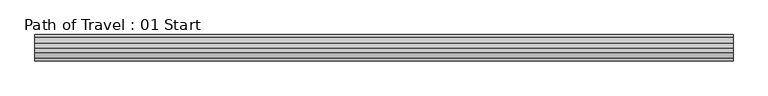
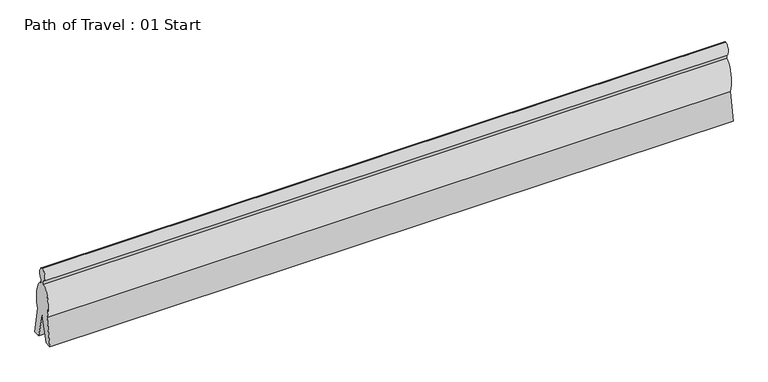
"""IFC4 building model written with IfcOpenShell, lengths in millimetres: proxy geometry, Path of Travel : 01 Start."""

import ifcopenshell
import ifcopenshell.guid

model = None  # the IFC model being written
_history = None  # IfcOwnerHistory: only IFC2X3 demands one
_inside = {}  # id of a spatial element -> (the spatial element, [elements in it])
_under = {}  # id of a project, library or spatial element -> (it, [spatial elements below it])
_declared = {}  # id of a project -> (the project, [libraries it declares])
_typed = {}  # id of a type object -> (the type object, [elements of that type])
_made_of = {}  # id of a material, layer set ... -> (it, [elements and type objects made of it])


def new_model(schema):
    """Start an empty IFC model of exactly this schema.

    Asked for "IFC4X3", IfcOpenShell would pick the latest addendum, in which some entities
    have other attributes; the version numbers below select the first issue.
    IFC2X3 requires an IfcOwnerHistory on every rooted entity: one is made here for all.
    """
    global model, _history
    if schema == "IFC4X3":
        model = ifcopenshell.file(schema_version=(4, 3, 0, 0))
    else:
        model = ifcopenshell.file(schema=schema)
    _inside.clear()
    _under.clear()
    _declared.clear()
    _typed.clear()
    _made_of.clear()
    _history = None
    if model.schema == "IFC2X3":
        org = make("IfcOrganization", Name="unknown")
        user = make(
            "IfcPersonAndOrganization",
            ThePerson=make("IfcPerson", FamilyName="unknown"),
            TheOrganization=org,
        )
        app = make(
            "IfcApplication",
            ApplicationDeveloper=org,
            Version="unknown",
            ApplicationFullName="unknown",
            ApplicationIdentifier="unknown",
        )
        _history = make(
            "IfcOwnerHistory",
            OwningUser=user,
            OwningApplication=app,
            ChangeAction="ADDED",
            CreationDate=0,
        )
    return model


def make(cls, **values):
    """One entity of the class cls with the attributes given. An attribute that is None is left unset."""
    return model.create_entity(
        cls, **{name: value for name, value in values.items() if value is not None}
    )


def rooted(cls, **values):
    """An entity with a GlobalId (a new one), such as an element, a storey or a relation."""
    return make(cls, GlobalId=ifcopenshell.guid.new(), OwnerHistory=_history, **values)


def si_unit(unit_type, name, prefix=None):
    """IfcSIUnit, for example si_unit("LENGTHUNIT", "METRE", prefix="MILLI")."""
    return make("IfcSIUnit", UnitType=unit_type, Prefix=prefix, Name=name)


def assignment(units):
    """IfcUnitAssignment: the units of a project."""
    return None if units is None else make("IfcUnitAssignment", Units=units)


def point(xyz):
    """IfcCartesianPoint."""
    return None if xyz is None else make("IfcCartesianPoint", Coordinates=xyz)


def direction(xyz):
    """IfcDirection."""
    return None if xyz is None else make("IfcDirection", DirectionRatios=xyz)


def frame(location, z_axis=None, x_axis=None):
    """IfcAxis2Placement3D, a coordinate frame: its origin and axes. An axis left out is left unset."""
    return make(
        "IfcAxis2Placement3D",
        Location=point(location),
        Axis=direction(z_axis),
        RefDirection=direction(x_axis),
    )


def origin():
    """The frame at (0, 0, 0) with its axes left unset."""
    return frame((0.0, 0.0, 0.0))


def place(relative_to, where):
    """IfcLocalPlacement: puts the frame where relative to a parent placement (None: the world)."""
    return make(
        "IfcLocalPlacement", PlacementRelTo=relative_to, RelativePlacement=where
    )


def context(
    kind, dimensions, precision=None, world=None, true_north=None, identifier=None
):
    """IfcGeometricRepresentationContext, for example the 3D "Model" context."""
    return make(
        "IfcGeometricRepresentationContext",
        ContextIdentifier=identifier,
        ContextType=kind,
        CoordinateSpaceDimension=dimensions,
        Precision=precision,
        WorldCoordinateSystem=world,
        TrueNorth=true_north,
    )


def project(units=None, contexts=None):
    """IfcProject with its units and contexts."""
    return rooted(
        "IfcProject",
        Name="project",
        RepresentationContexts=contexts,
        UnitsInContext=assignment(units),
    )


def spatial(cls, under=None, at=None, **own):
    """A site, building, storey or space (cls), placed at a placement, below another one or the project."""
    s = rooted(cls, ObjectPlacement=at, **own)
    if under is not None:
        _under.setdefault(under.id(), (under, []))[1].append(s)
    return s


def ellipse_curve(where, semi_axis1, semi_axis2):
    """IfcEllipse in the frame where."""
    return make(
        "IfcEllipse", Position=where, SemiAxis1=semi_axis1, SemiAxis2=semi_axis2
    )


def trimmed(basis, trim1, trim2, sense, master):
    """IfcTrimmedCurve: the piece of a basis curve between two trims."""
    return make(
        "IfcTrimmedCurve",
        BasisCurve=basis,
        Trim1=trim1,
        Trim2=trim2,
        SenseAgreement=sense,
        MasterRepresentation=master,
    )


def shape(context_of_items, identifier, shape_type, items):
    """IfcShapeRepresentation: the items that make up one representation, for example the "Body"."""
    return make(
        "IfcShapeRepresentation",
        ContextOfItems=context_of_items,
        RepresentationIdentifier=identifier,
        RepresentationType=shape_type,
        Items=items,
    )


def source(mapping_origin, context_of_items, identifier, shape_type, items):
    """IfcRepresentationMap: a shape defined once, which mapped items show again and again."""
    return make(
        "IfcRepresentationMap",
        MappingOrigin=mapping_origin,
        MappedRepresentation=shape(context_of_items, identifier, shape_type, items),
    )


def transform(
    local_origin,
    x_axis=None,
    y_axis=None,
    z_axis=None,
    scale=None,
    scale2=None,
    scale3=None,
    uniform=True,
):
    """IfcCartesianTransformationOperator3D, or its non-uniform kind. x_axis, y_axis, z_axis: its Axis1, 2, 3."""
    if uniform:
        return make(
            "IfcCartesianTransformationOperator3D",
            Axis1=direction(x_axis),
            Axis2=direction(y_axis),
            LocalOrigin=point(local_origin),
            Scale=scale,
            Axis3=direction(z_axis),
        )
    return make(
        "IfcCartesianTransformationOperator3DnonUniform",
        Axis1=direction(x_axis),
        Axis2=direction(y_axis),
        LocalOrigin=point(local_origin),
        Scale=scale,
        Axis3=direction(z_axis),
        Scale2=scale2,
        Scale3=scale3,
    )


def mapped(mapping_source, mapping_target):
    """IfcMappedItem: shows the shape of a source again, moved by a transform."""
    return make(
        "IfcMappedItem", MappingSource=mapping_source, MappingTarget=mapping_target
    )


def made_of(thing, what):
    """Note that an element or type object is made of a material, layer set ...; save() writes the relation."""
    if what is not None:
        _made_of.setdefault(what.id(), (what, []))[1].append(thing)
    return thing


def element(
    cls,
    number,
    at=None,
    inside=None,
    cuts=None,
    type_object=None,
    material=None,
    context=None,
    identifier="Body",
    shape_type=None,
    held_by="IfcProductDefinitionShape",
    body=None,
    shapes=None,
    **own,
):
    """One element of the class cls, such as IfcWall. Its Tag is "e" and its number.

    at: its placement. inside: the storey or other place that contains it. cuts: it is an
    opening in that element (IfcRelVoidsElement). A single representation is given by context,
    identifier, shape_type and body (its items); several are given by shapes. held_by: the class
    of the entity that holds the representations. save() writes the other relations.
    """
    e = rooted(cls, Tag="e%d" % number, ObjectPlacement=at, **own)
    if body is not None:
        shapes = [shape(context, identifier, shape_type, body)]
    if shapes is not None:
        e.Representation = make(held_by, Representations=shapes)
    if inside is not None:
        _inside.setdefault(inside.id(), (inside, []))[1].append(e)
    if cuts is not None:
        rooted(
            "IfcRelVoidsElement", RelatingBuildingElement=cuts, RelatedOpeningElement=e
        )
    if type_object is not None:
        _typed.setdefault(type_object.id(), (type_object, []))[1].append(e)
    return made_of(e, material)


def aggregate(whole, parts):
    """IfcRelAggregates: a whole, such as a stair, and the parts it consists of."""
    return rooted("IfcRelAggregates", RelatingObject=whole, RelatedObjects=parts)


def save(model, path):
    """Write the relations noted so far, then the file.

    IfcRelAggregates (storeys below a building ...), IfcRelContainedInSpatialStructure (elements
    in a storey), IfcRelDefinesByType, IfcRelAssociatesMaterial and IfcRelDeclares: one each for
    every whole, place, type object, material and project.
    """
    for whole, parts in _under.values():
        aggregate(whole, parts)
    for where, things in _inside.values():
        rooted(
            "IfcRelContainedInSpatialStructure",
            RelatedElements=things,
            RelatingStructure=where,
        )
    for kind, things in _typed.values():
        rooted("IfcRelDefinesByType", RelatedObjects=things, RelatingType=kind)
    for what, things in _made_of.values():
        rooted("IfcRelAssociatesMaterial", RelatedObjects=things, RelatingMaterial=what)
    for by, libraries in _declared.values():
        rooted("IfcRelDeclares", RelatingContext=by, RelatedDefinitions=libraries)
    model.write(path)


def plane_surface(at):
    """IfcPlane: the flat surface through the origin of the frame at, square to its z axis."""
    return make("IfcPlane", Position=at)


def extruded_surface(curve, direction_of_extrusion, depth):
    """IfcSurfaceOfLinearExtrusion: the curve pushed along a direction by depth."""
    return make(
        "IfcSurfaceOfLinearExtrusion",
        SweptCurve=make("IfcArbitraryOpenProfileDef", ProfileType="CURVE", Curve=curve),
        ExtrudedDirection=direction(direction_of_extrusion),
        Depth=depth,
    )


def advanced_brep(points, edges, surfaces, faces):
    """IfcAdvancedBrep: a solid bounded by faces that lie on surfaces and meet in shared edges.

    An edge is (start, end): straight between two places in points (the first is 0);
    or (start, end, curve); or (start, end, curve, False) where it runs against its curve.
    A face is (place in surfaces, loops), or (place, loops, False) where it looks against
    its surface's normal. A loop lists edges by number (the first is 1), with a minus sign
    where the edge is run from its end to its start. The first loop is the outer one.
    """
    corners = [point(p) for p in points]
    vertices = [make("IfcVertexPoint", VertexGeometry=c) for c in corners]
    made = []
    for start, end, *more in edges:
        made.append(
            make(
                "IfcEdgeCurve",
                EdgeStart=vertices[start],
                EdgeEnd=vertices[end],
                EdgeGeometry=more[0] if more else make("IfcPolyline", Points=[corners[start], corners[end]]),
                SameSense=more[1] if len(more) > 1 else True,
            )
        )
    hull = []
    for where, loops, *sense in faces:
        bounds = []
        for j, loop in enumerate(loops):
            ring = [make("IfcOrientedEdge", EdgeElement=made[abs(k) - 1], Orientation=k > 0) for k in loop]
            bounds.append(
                make(
                    "IfcFaceOuterBound" if j == 0 else "IfcFaceBound",
                    Bound=make("IfcEdgeLoop", EdgeList=ring),
                    Orientation=True,
                )
            )
        hull.append(make("IfcAdvancedFace", Bounds=bounds, FaceSurface=surfaces[where], SameSense=sense[0] if sense else True))
    return make("IfcAdvancedBrep", Outer=make("IfcClosedShell", CfsFaces=hull))


def path_of_travel_01_start_5b2d4024(model_context):
    return source(origin(), model_context, "Body", "AdvancedBrep", [
        advanced_brep(
        [(227.5554837, 0.0, 1727.2), (227.5554837, 42.9018657, 1436.6534209), (227.5554837, 42.9018657, 1363.4763406), (227.5554837, 184.1186263, 643.4144547), (227.5554837, 297.5699544, 0.0), (227.5554837, 145.6574193, 0.0), (227.5554837, 0.0, 584.2), (227.5554837, -145.6574193, 0.0), (227.5554837, -297.5699544, 0.0), (227.5554837, -184.1186263, 643.4144547), (227.5554837, -42.9018657, 1363.4763406), (227.5554837, -42.9018657, 1436.6534209), (15899.3554837, 0.0, 1727.2), (15899.3554837, -42.9018657, 1436.6534209), (15899.3554837, -42.9018657, 1363.4763406), (15899.3554837, -184.1186263, 643.4144547), (15899.3554837, -297.5699544, 0.0), (15899.3554837, -145.6574193, 0.0), (15899.3554837, 0.0, 584.2), (15899.3554837, 145.6574193, 0.0), (15899.3554837, 297.5699544, 0.0), (15899.3554837, 184.1186263, 643.4144547), (15899.3554837, 42.9018657, 1363.4763406), (15899.3554837, 42.9018657, 1436.6534209)],
        [
            (0, 1, ellipse_curve(frame((227.5554837, 0.0, 1574.8), z_axis=(-1.0, 0.0, 0.0), x_axis=(0.0, 0.0, 1.0)), 152.4, 101.6)),
            (1, 2),
            (2, 3, ellipse_curve(frame((227.5554837, 0.0, 914.4), z_axis=(-1.0, 0.0, 0.0), x_axis=(0.0, 0.0, -1.0)), 457.2, 228.6)),
            (3, 4),
            (4, 5),
            (5, 6),
            (6, 7),
            (7, 8),
            (8, 9),
            (9, 10, ellipse_curve(frame((227.5554837, 0.0, 914.4), z_axis=(-1.0, 0.0, 0.0), x_axis=(0.0, 0.0, -1.0)), 457.2, 228.6)),
            (10, 11),
            (11, 0, ellipse_curve(frame((227.5554837, 0.0, 1574.8), z_axis=(-1.0, 0.0, 0.0), x_axis=(0.0, 0.0, 1.0)), 152.4, 101.6)),
            (12, 13, ellipse_curve(frame((15899.3554837, 0.0, 1574.8), z_axis=(1.0, 0.0, 0.0), x_axis=(0.0, 0.0, 1.0)), 152.4, 101.6)),
            (13, 14),
            (14, 15, ellipse_curve(frame((15899.3554837, 0.0, 914.4), z_axis=(1.0, 0.0, 0.0), x_axis=(0.0, 0.0, -1.0)), 457.2, 228.6)),
            (15, 16),
            (16, 17),
            (17, 18),
            (18, 19),
            (19, 20),
            (20, 21),
            (21, 22, ellipse_curve(frame((15899.3554837, 0.0, 914.4), z_axis=(1.0, 0.0, 0.0), x_axis=(0.0, 0.0, -1.0)), 457.2, 228.6)),
            (22, 23),
            (23, 12, ellipse_curve(frame((15899.3554837, 0.0, 1574.8), z_axis=(1.0, 0.0, 0.0), x_axis=(0.0, 0.0, 1.0)), 152.4, 101.6)),
            (11, 13),
            (12, 0),
            (10, 14),
            (9, 15),
            (8, 16),
            (7, 17),
            (6, 18),
            (5, 19),
            (4, 20),
            (3, 21),
            (2, 22),
            (1, 23),
        ],
        [
            plane_surface(frame((227.5554837, 0.0, 0.0), z_axis=(-1.0, 0.0, 0.0), x_axis=(0.0, 0.0, 1.0))),
            plane_surface(frame((15899.3554837, 0.0, 0.0), z_axis=(1.0, 0.0, 0.0), x_axis=(0.0, 0.0, 1.0))),
            extruded_surface(trimmed(ellipse_curve(frame((227.5554837, 0.0, 1574.8), z_axis=(1.0, 0.0, 0.0), x_axis=(0.0, 0.0, 1.0)), 152.4, 101.6), [point((227.5554837, 0.0, 1727.2))], [point((227.5554837, -42.9018657, 1436.6534209))], True, "CARTESIAN"), (15671.8, 0.0, 0.0), 15671.8),
            plane_surface(frame((227.5554837, -42.9018657, 1436.6534209), z_axis=(0.0, -1.0, 0.0), x_axis=(1.0, 0.0, 0.0))),
            extruded_surface(trimmed(ellipse_curve(frame((227.5554837, 0.0, 914.4), z_axis=(1.0, 0.0, 0.0), x_axis=(0.0, 0.0, -1.0)), 457.2, 228.6), [point((227.5554837, -42.9018657, 1363.4763406))], [point((227.5554837, -184.1186263, 643.4144547))], True, "CARTESIAN"), (15671.8, 0.0, 0.0), 15671.8),
            plane_surface(frame((227.5554837, -184.1186263, 643.4144547), z_axis=(0.0, -0.9848077530122078, 0.17364817766693205), x_axis=(1.0, 0.0, 0.0))),
            plane_surface(frame((227.5554837, -297.5699544, 0.0), z_axis=(0.0, 0.0, -1.0), x_axis=(1.0, 0.0, 0.0))),
            plane_surface(frame((227.5554837, -145.6574193, 0.0), z_axis=(0.0, 0.9702957262760199, -0.2419218955995739), x_axis=(1.0, 0.0, 0.0))),
            plane_surface(frame((227.5554837, 0.0, 584.2), z_axis=(0.0, -0.9702957262759961, -0.24192189559966923), x_axis=(1.0, 0.0, 0.0))),
            plane_surface(frame((227.5554837, 145.6574193, 0.0), z_axis=(0.0, 0.0, -1.0), x_axis=(1.0, 0.0, 0.0))),
            plane_surface(frame((227.5554837, 297.5699544, 0.0), z_axis=(0.0, 0.984807753012208, 0.17364817766693066), x_axis=(1.0, 0.0, 0.0))),
            extruded_surface(trimmed(ellipse_curve(frame((227.5554837, 0.0, 914.4), z_axis=(1.0, 0.0, 0.0), x_axis=(0.0, 0.0, -1.0)), 457.2, 228.6), [point((227.5554837, 184.1186263, 643.4144547))], [point((227.5554837, 42.9018657, 1363.4763406))], True, "CARTESIAN"), (15671.8, 0.0, 0.0), 15671.8),
            plane_surface(frame((227.5554837, 42.9018657, 1363.4763406), z_axis=(0.0, 1.0, 0.0), x_axis=(1.0, 0.0, 0.0))),
            extruded_surface(trimmed(ellipse_curve(frame((227.5554837, 0.0, 1574.8), z_axis=(1.0, 0.0, 0.0), x_axis=(0.0, 0.0, 1.0)), 152.4, 101.6), [point((227.5554837, 42.9018657, 1436.6534209))], [point((227.5554837, 0.0, 1727.2))], True, "CARTESIAN"), (15671.8, 0.0, 0.0), 15671.8),
        ],
        [
            (0, [[1, 2, 3, 4, 5, 6, 7, 8, 9, 10, 11, 12]]),
            (1, [[13, 14, 15, 16, 17, 18, 19, 20, 21, 22, 23, 24]]),
            (2, [[25, -13, 26, -12]]),
            (3, [[27, -14, -25, -11]]),
            (4, [[28, -15, -27, -10]]),
            (5, [[29, -16, -28, -9]]),
            (6, [[30, -17, -29, -8]]),
            (7, [[31, -18, -30, -7]]),
            (8, [[32, -19, -31, -6]]),
            (9, [[33, -20, -32, -5]]),
            (10, [[34, -21, -33, -4]]),
            (11, [[35, -22, -34, -3]]),
            (12, [[36, -23, -35, -2]]),
            (13, [[-26, -24, -36, -1]]),
        ],
    ),
    ])


if __name__ == "__main__":
    model = new_model("IFC4")
    model_context = context("Model", 3, world=origin())
    ifc_project = project(units=[si_unit("LENGTHUNIT", "METRE", prefix="MILLI")], contexts=[model_context])
    site = spatial("IfcSite", under=ifc_project)
    building = spatial("IfcBuilding", under=site)
    placement = place(None, origin())
    path_of_travel_01_start_shape = path_of_travel_01_start_5b2d4024(model_context)
    element("IfcBuildingElementProxy", 1, Name="Path of Travel : 01 Start", ObjectType="Path of Travel : 01 Start", at=placement, inside=building, context=model_context, shape_type="MappedRepresentation", body=[
        mapped(path_of_travel_01_start_shape, transform((0.0, 0.0, 0.0), x_axis=(1.0, 0.0, 0.0), y_axis=(0.0, 1.0, 0.0), z_axis=(0.0, 0.0, 1.0))),
    ])
    save(model, "model.ifc")

# Revit data of these elements
# Type "Path of Travel : 01 Start"
#   Path of Egress [instance default] = 4' - 0"
#   built-in parameter 1001306 [instance default] = 4 (stored number, unit not read)
#   Dot at Start = yes
#   Arrow in Middle = yes
#   Arrow at End = no
#   Egress Path = none
# Element 1 (IfcBuildingElementProxy, "Path of Travel : 01 Start")
#   Path of Egress = 51' - 5"
#   built-in parameter 1001306 = 51.4167 (stored number, unit not read)
#   Materials on its faces: "Egress Path Solid"
# Materials
#   "Egress Path Solid": class "Unassigned", colour RGB 255 128 64, transparency 0.75, Comments = "Rendering appearance not upgraded "
